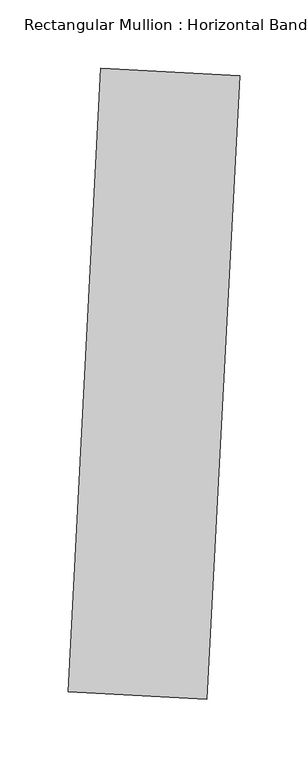
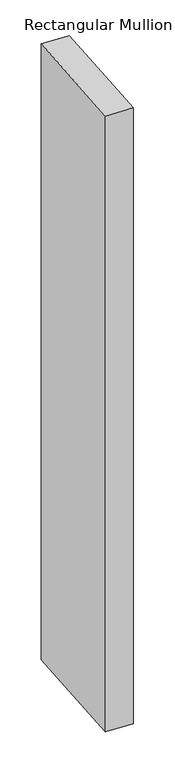
"""IFC4 building model written with IfcOpenShell, lengths in millimetres: member geometry, Rectangular Mullion : Horizontal Band."""

from ifc_helpers import new_model, si_unit, frame, origin, place, context, project, spatial, polyline, outline, extrude, source, transform, mapped, element, save


def rectangular_mullion_horizontal_band_9c283acf(model_context):
    return source(origin(), model_context, "Body", "SweptSolid", [
        extrude(outline(polyline([(62.69438, 301.8280451), (38.7663808, -154.7453782), (-62.69438, -149.4280451), (-38.7663808, 307.1453782), (62.69438, 301.8280451)])), frame((0.0, 0.0, -2437.4403502), z_axis=(0.0, 0.0, 1.0), x_axis=(1.0, 0.0, 0.0)), (0.0, 0.0, 1.0), 2437.4403502),
    ])


if __name__ == "__main__":
    model = new_model("IFC4")
    model_context = context("Model", 3, world=origin())
    ifc_project = project(units=[si_unit("LENGTHUNIT", "METRE", prefix="MILLI")], contexts=[model_context])
    site = spatial("IfcSite", under=ifc_project)
    building = spatial("IfcBuilding", under=site)
    placement = place(None, origin())
    rectangular_mullion_horizontal_band_shape = rectangular_mullion_horizontal_band_9c283acf(model_context)
    element("IfcMember", 1, ObjectType="Rectangular Mullion : Horizontal Band", at=placement, inside=building, context=model_context, shape_type="MappedRepresentation", body=[
        mapped(rectangular_mullion_horizontal_band_shape, transform((0.0, 0.0, 0.0), x_axis=(1.0, 0.0, 0.0), y_axis=(0.0, 1.0, 0.0), z_axis=(0.0, 0.0, 1.0))),
    ])
    save(model, "model.ifc")

# Revit data of these elements
# Type "Rectangular Mullion : Horizontal Band"
#   built-in parameter 1007351 = 0.25 (stored number, unit not read)
#   built-in parameter 1007304 = 1.5 (stored number, unit not read)
#   built-in parameter 1007301 = 0.166667 (stored number, unit not read)
#   built-in parameter 1007300 = 0.166667 (stored number, unit not read)
# Element 1 (IfcMember, "Rectangular Mullion : Horizontal Band")
#   Materials on its faces: "Aluminum"
# Materials
#   "Aluminum": class "Metal", colour RGB 247 247 247, transparency 0, Description = "Aluminum 6061", Cost = 0
